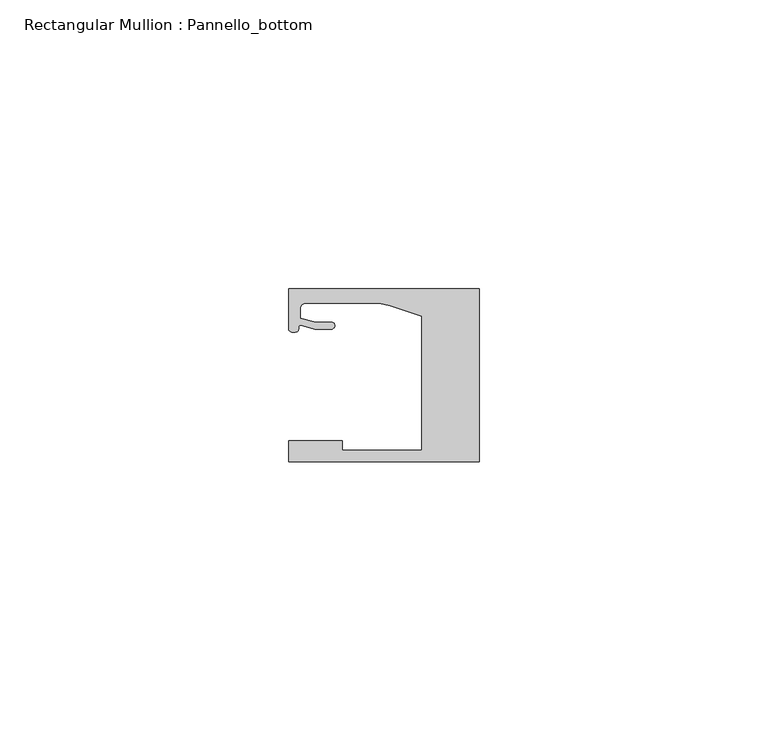
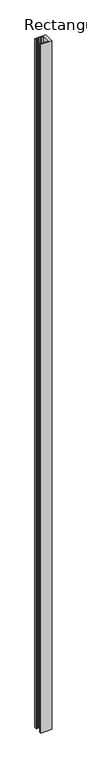
"""IFC4 building model written with IfcOpenShell, lengths in millimetres: member geometry, Rectangular Mullion : Pannello_bottom."""

from ifc_helpers import new_model, si_unit, frame, origin, place, context, project, spatial, polyline, circle_curve, source, transform, mapped, element, save
from ifc_brep_helpers import plane_surface, cylinder_surface, revolved_surface, extruded_surface, spline_curve, advanced_brep


def rectangular_mullion_pannello_bottom_7ab77e3f(model_context):
    return source(origin(), model_context, "Body", "AdvancedBrep", [
        advanced_brep(
        [(-33.0, -15.0, 0.0), (0.0, -15.0, 0.0), (0.0, 15.0, 0.0), (-33.0000135, 15.0, 0.0), (-33.0000135, 8.0000472, 0.0), (-30.9223017, 8.6490241, 0.0), (-28.4999305, 7.9999523, 0.0), (-25.59998, 7.9999523, 0.0), (-25.59998, 9.1999523, 0.0), (-28.3419477, 9.1999523, 0.0), (-31.0, 9.9121746, 0.0), (-31.0, 11.4999419, 0.0), (-30.0000002, 12.4999419, 0.0), (-18.5493024, 12.4999438, 0.0), (-15.4591336, 12.0105099, 0.0), (-9.9999723, 10.2367227, 0.0), (-9.9999723, -13.0000004, 0.0), (-23.700041, -13.0000004, 0.0), (-23.700041, -11.3000004, 0.0), (-33.0, -11.3000004, 0.0), (-33.0, -15.0, -2173.9999729), (-33.0, -11.3000004, -2173.9999729), (-23.700041, -11.3000004, -2173.9999729), (-23.700041, -13.0000004, -2173.9999729), (-9.9999723, -13.0000004, -2173.9999729), (-9.9999723, 10.2367227, -2173.9999729), (-15.4591336, 12.0105099, -2173.9999729), (-18.5493024, 12.4999438, -2173.9999729), (-30.0000002, 12.4999419, -2173.9999729), (-31.0, 11.4999419, -2173.9999729), (-31.0, 9.9121746, -2173.9999729), (-28.3419477, 9.1999523, -2173.9999729), (-25.59998, 9.1999523, -2173.9999729), (-25.59998, 7.9999523, -2173.9999729), (-28.4999305, 7.9999523, -2173.9999729), (-30.9223017, 8.6490241, -2173.9999729), (-33.0000135, 8.0000472, -2173.9999729), (-33.0000135, 15.0, -2173.9999729), (0.0, 15.0, -2173.9999729), (0.0, -15.0, -2173.9999729)],
        [
            (0, 1),
            (1, 2),
            (2, 3),
            (3, 4),
            (4, 5, spline_curve(3, [(-33.0000135, 8.0000472, 0.0), (-33.0000135, 7.457047519, 0.0), (-32.262327879, 7.456527435, 0.0), (-31.357433266, 7.563996614, 0.0), (-31.305645054, 7.690065204, 0.0), (-31.298563602, 8.366228555, 0.0), (-31.312054066, 8.717747958, 0.0), (-30.9223017, 8.6490241, 0.0)], [4, 2, 2, 4], [0.0, 0.0027053965905959043, 0.0058611956533709, 0.007702013405570312])),
            (5, 6),
            (6, 7),
            (7, 8, circle_curve(frame((-25.59998, 8.5999523, 0.0), z_axis=(0.0, 0.0, 1.0), x_axis=(0.0, 1.0, 0.0)), 0.6)),
            (8, 9),
            (9, 10),
            (10, 11),
            (11, 12, circle_curve(frame((-30.0, 11.4999419, 0.0), z_axis=(0.0, 0.0, -1.0), x_axis=(0.0, 1.0, 0.0)), 1.0)),
            (12, 13),
            (13, 14, circle_curve(frame((-18.5493007, 2.4999438, 0.0), z_axis=(0.0, 0.0, -1.0), x_axis=(0.0, 1.0, 0.0)), 10.0)),
            (14, 15),
            (15, 16),
            (16, 17),
            (17, 18),
            (18, 19),
            (19, 0),
            (20, 21),
            (21, 22),
            (22, 23),
            (23, 24),
            (24, 25),
            (25, 26),
            (26, 27, circle_curve(frame((-18.5493007, 2.4999438, -2173.9999729), z_axis=(0.0, 0.0, 1.0), x_axis=(0.0, 1.0, 0.0)), 10.0)),
            (27, 28),
            (28, 29, circle_curve(frame((-30.0, 11.4999419, -2173.9999729), z_axis=(0.0, 0.0, 1.0), x_axis=(0.0, 1.0, 0.0)), 1.0)),
            (29, 30),
            (30, 31),
            (31, 32),
            (32, 33, circle_curve(frame((-25.59998, 8.5999523, -2173.9999729), z_axis=(0.0, 0.0, -1.0), x_axis=(0.0, 1.0, 0.0)), 0.6)),
            (33, 34),
            (34, 35),
            (35, 36, spline_curve(3, [(-30.9223017, 8.6490241, -2173.9999729), (-31.312054066, 8.717747958, -2173.9999729), (-31.298563602, 8.366228555, -2173.9999729), (-31.305645054, 7.690065204, -2173.9999729), (-31.357433266, 7.563996614, -2173.9999729), (-32.262327879, 7.456527435, -2173.9999729), (-33.0000135, 7.457047519, -2173.9999729), (-33.0000135, 8.0000472, -2173.9999729)], [4, 2, 2, 4], [0.0, 0.001840817752199412, 0.004996616814974408, 0.007702013405570312])),
            (36, 37),
            (37, 38),
            (38, 39),
            (39, 20),
            (0, 20),
            (39, 1),
            (38, 2),
            (37, 3),
            (36, 4),
            (35, 5),
            (34, 6),
            (33, 7),
            (32, 8),
            (31, 9),
            (30, 10),
            (29, 11),
            (28, 12),
            (27, 13),
            (26, 14),
            (25, 15),
            (24, 16),
            (23, 17),
            (22, 18),
            (21, 19),
        ],
        [
            plane_surface(frame((0.0, -36.2491502, 0.0), z_axis=(0.0, 0.0, 1.0), x_axis=(-1.0, 0.0, 0.0))),
            plane_surface(frame((0.0, -36.2491502, -2173.9999729), z_axis=(0.0, 0.0, -1.0), x_axis=(-1.0, 0.0, 0.0))),
            plane_surface(frame((-33.0, -15.0, 0.0), z_axis=(0.0, -1.0, 0.0), x_axis=(0.0, 0.0, -1.0))),
            plane_surface(frame((0.0, -15.0, 0.0), z_axis=(1.0, 0.0, 0.0), x_axis=(0.0, 0.0, -1.0))),
            plane_surface(frame((0.0, 15.0, 0.0), z_axis=(0.0, 1.0, 0.0), x_axis=(0.0, 0.0, -1.0))),
            plane_surface(frame((-33.0000135, 15.0, 0.0), z_axis=(-1.0, 0.0, 0.0), x_axis=(0.0, 0.0, -1.0))),
            extruded_surface(spline_curve(3, [(-33.0000135, 8.0000472, -2173.9999729), (-33.0000135, 7.457047519, -2173.9999729), (-32.262327879, 7.456527435, -2173.9999729), (-31.357433266, 7.563996614, -2173.9999729), (-31.305645054, 7.690065204, -2173.9999729), (-31.298563602, 8.366228555, -2173.9999729), (-31.312054066, 8.717747958, -2173.9999729), (-30.9223017, 8.6490241, -2173.9999729)], [4, 2, 2, 4], [0.0, 0.0027053965905959043, 0.0058611956533709, 0.007702013405570312]), (0.0, 0.0, 2173.9999729), 2173.9999729),
            plane_surface(frame((-30.9223017, 8.6490241, 0.0), z_axis=(-0.25881883200192934, -0.9659258833891746, 0.0), x_axis=(0.0, 0.0, -1.0))),
            plane_surface(frame((-28.4999305, 7.9999523, 0.0), z_axis=(0.0, -1.0, 0.0), x_axis=(0.0, 0.0, -1.0))),
            cylinder_surface(frame((-25.59998, 8.5999523, 0.0), z_axis=(0.0, 0.0, 1.0), x_axis=(0.0, 1.0, 0.0)), 0.6),
            plane_surface(frame((-25.59998, 9.1999523, 0.0), z_axis=(0.0, 1.0, 0.0), x_axis=(0.0, 0.0, -1.0))),
            plane_surface(frame((-28.3419477, 9.1999523, 0.0), z_axis=(0.25881883204288636, 0.9659258833782002, 0.0), x_axis=(0.0, 0.0, -1.0))),
            plane_surface(frame((-31.0, 9.9121746, 0.0), z_axis=(1.0, 0.0, 0.0), x_axis=(0.0, 0.0, -1.0))),
            revolved_surface(polyline([(-30.0, 12.4999419, -2173.9999729), (-30.0, 12.4999419, 0.0)]), (-30.0, 11.4999419, 0.0), (0.0, 0.0, -1.0)),
            plane_surface(frame((-30.0000002, 12.4999419, 0.0), z_axis=(1.6923026533778639e-07, -0.9999999999999858, 0.0), x_axis=(0.0, 0.0, -1.0))),
            revolved_surface(polyline([(-18.5493007, 12.4999438, -2173.9999729), (-18.5493007, 12.4999438, 0.0)]), (-18.5493007, 2.4999438, 0.0), (0.0, 0.0, -1.0)),
            plane_surface(frame((-15.4591336, 12.0105099, 0.0), z_axis=(-0.30901670911956314, -0.9510566089801992, 0.0), x_axis=(0.0, 0.0, -1.0))),
            plane_surface(frame((-9.9999723, 10.2367227, 0.0), z_axis=(-1.0, 0.0, 0.0), x_axis=(0.0, 0.0, -1.0))),
            plane_surface(frame((-9.9999723, -13.0000004, 0.0), z_axis=(0.0, 1.0, 0.0), x_axis=(0.0, 0.0, -1.0))),
            plane_surface(frame((-23.700041, -13.0000004, 0.0), z_axis=(1.0, 0.0, 0.0), x_axis=(0.0, 0.0, -1.0))),
            plane_surface(frame((-23.700041, -11.3000004, 0.0), z_axis=(0.0, 1.0, 0.0), x_axis=(0.0, 0.0, -1.0))),
            plane_surface(frame((-33.0, -11.3000004, 0.0), z_axis=(-1.0, 0.0, 0.0), x_axis=(0.0, 0.0, -1.0))),
        ],
        [
            (0, [[1, 2, 3, 4, 5, 6, 7, 8, 9, 10, 11, 12, 13, 14, 15, 16, 17, 18, 19, 20]]),
            (1, [[21, 22, 23, 24, 25, 26, 27, 28, 29, 30, 31, 32, 33, 34, 35, 36, 37, 38, 39, 40]]),
            (2, [[-1, 41, -40, 42]]),
            (3, [[-2, -42, -39, 43]]),
            (4, [[-3, -43, -38, 44]]),
            (5, [[-4, -44, -37, 45]]),
            (6, [[-5, -45, -36, 46]]),
            (7, [[-6, -46, -35, 47]]),
            (8, [[-7, -47, -34, 48]]),
            (9, [[-8, -48, -33, 49]]),
            (10, [[-9, -49, -32, 50]]),
            (11, [[-10, -50, -31, 51]]),
            (12, [[-11, -51, -30, 52]]),
            (13, [[-12, -52, -29, 53]]),
            (14, [[-13, -53, -28, 54]]),
            (15, [[-14, -54, -27, 55]]),
            (16, [[-15, -55, -26, 56]]),
            (17, [[-16, -56, -25, 57]]),
            (18, [[-17, -57, -24, 58]]),
            (19, [[-18, -58, -23, 59]]),
            (20, [[-19, -59, -22, 60]]),
            (21, [[-20, -60, -21, -41]]),
        ],
    ),
    ])


if __name__ == "__main__":
    model = new_model("IFC4")
    model_context = context("Model", 3, world=origin())
    ifc_project = project(units=[si_unit("LENGTHUNIT", "METRE", prefix="MILLI")], contexts=[model_context])
    site = spatial("IfcSite", under=ifc_project)
    building = spatial("IfcBuilding", under=site)
    placement = place(None, origin())
    rectangular_mullion_pannello_bottom_shape = rectangular_mullion_pannello_bottom_7ab77e3f(model_context)
    element("IfcMember", 1, ObjectType="Rectangular Mullion : Pannello_bottom", at=placement, inside=building, context=model_context, shape_type="MappedRepresentation", body=[
        mapped(rectangular_mullion_pannello_bottom_shape, transform((0.0, 0.0, 0.0), x_axis=(1.0, 0.0, 0.0), y_axis=(0.0, 1.0, 0.0), z_axis=(0.0, 0.0, 1.0))),
    ])
    save(model, "model.ifc")

# Revit data of these elements
# Type "Rectangular Mullion : Pannello_bottom"
#   built-in parameter 1007322 = 0.0984252 (stored number, unit not read)
#   built-in parameter 1007321 = 0.0328083 (stored number, unit not read)
#   built-in parameter 1007320 = 0 (stored number, unit not read)
